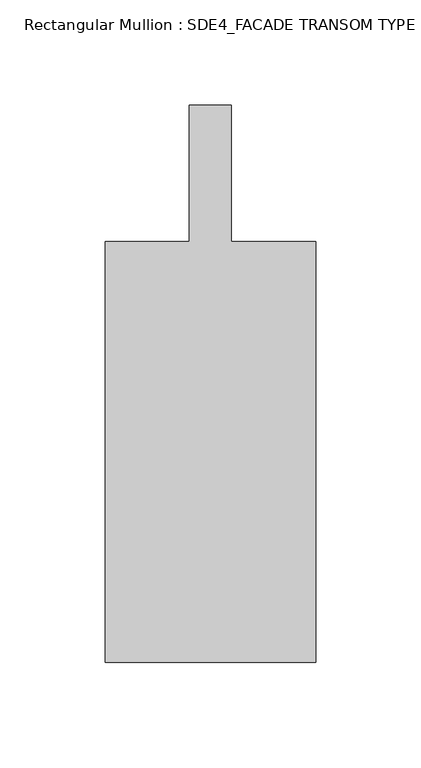
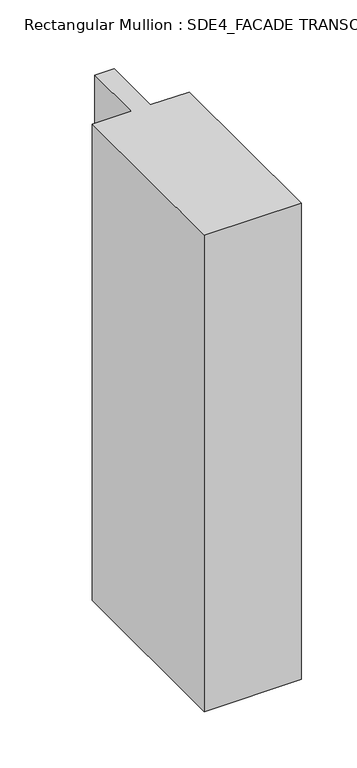
"""IFC4 building model written with IfcOpenShell, lengths in millimetres: member geometry, Rectangular Mullion : SDE4_FACADE TRANSOM TYPE 2."""

from ifc_helpers import new_model, si_unit, frame, origin, place, context, project, spatial, polyline, outline, extrude, source, transform, mapped, element, save


def rectangular_mullion_sde4_facade_transom_type_2_31aa32d0(model_context):
    return source(origin(), model_context, "Body", "SweptSolid", [
        extrude(outline(polyline([(50.0, -132.5), (-50.0, -132.5), (-50.0, 67.5), (-10.0, 67.5), (-10.0, 132.5), (10.0, 132.5), (10.0, 67.5), (50.0, 67.5), (50.0, -132.5)])), frame((0.0, 0.0, -520.3277581), z_axis=(0.0, 0.0, 1.0), x_axis=(1.0, 0.0, 0.0)), (0.0, 0.0, 1.0), 520.3277581),
    ])


if __name__ == "__main__":
    model = new_model("IFC4")
    model_context = context("Model", 3, world=origin())
    ifc_project = project(units=[si_unit("LENGTHUNIT", "METRE", prefix="MILLI")], contexts=[model_context])
    site = spatial("IfcSite", under=ifc_project)
    building = spatial("IfcBuilding", under=site)
    placement = place(None, origin())
    rectangular_mullion_sde4_facade_transom_type_2_shape = rectangular_mullion_sde4_facade_transom_type_2_31aa32d0(model_context)
    element("IfcMember", 1, ObjectType="Rectangular Mullion : SDE4_FACADE TRANSOM TYPE 2", at=placement, inside=building, context=model_context, shape_type="MappedRepresentation", body=[
        mapped(rectangular_mullion_sde4_facade_transom_type_2_shape, transform((0.0, 0.0, 0.0), x_axis=(1.0, 0.0, 0.0), y_axis=(0.0, 1.0, 0.0), z_axis=(0.0, 0.0, 1.0))),
    ])
    save(model, "model.ifc")

# Revit data of these elements
# Type "Rectangular Mullion : SDE4_FACADE TRANSOM TYPE 2"
#   built-in parameter 1007322 = 0.869423 (stored number, unit not read)
#   built-in parameter 1007321 = 0.164042 (stored number, unit not read)
#   built-in parameter 1007320 = 0.164042 (stored number, unit not read)
